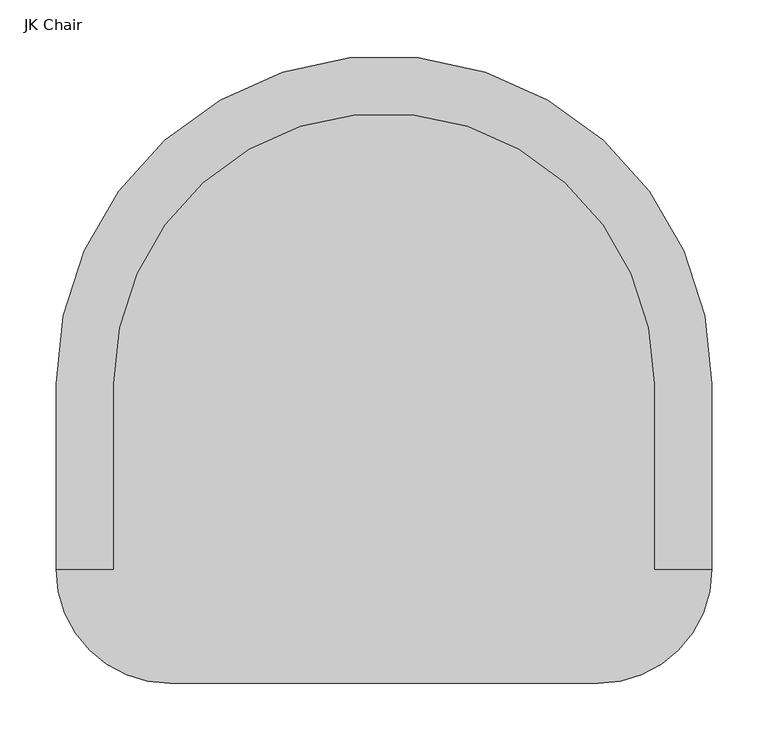
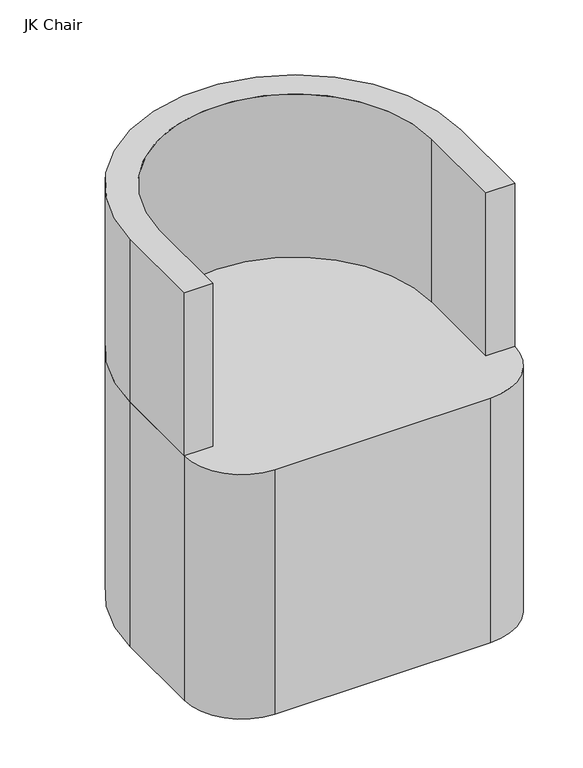
"""IFC4 building model written with IfcOpenShell, lengths in millimetres: furniture geometry, JK Chair : Recpt Chair."""

from ifc_helpers import new_model, si_unit, point, frame, frame_2d, origin, origin_with_axes, place, context, project, spatial, polyline, circle_curve, trimmed, segment, composite_curve, outline, extrude, source, transform, mapped, element, save


def jk_chair_91173c26(model_context):
    return source(origin(), model_context, "Body", "SweptSolid", [
        extrude(outline(composite_curve([segment(polyline([(-303.2426335, -131.5544704), (-354.0426335, -131.5544704), (-354.0426335, 33.5455296)]), True, "CONTINUOUS"), segment(trimmed(circle_curve(frame_2d((-61.9426335, 33.5455296)), 292.1), [point((-354.0426335, 33.5455296))], [point((230.1573665, 33.5455296))], False, "CARTESIAN"), True, "CONTINUOUS"), segment(polyline([(230.1573665, 33.5455296), (230.1573665, -131.5544704), (179.3573665, -131.5544704), (179.3573665, 33.5455296)]), True, "CONTINUOUS"), segment(trimmed(circle_curve(frame_2d((-61.9426335, 33.5455296)), 241.3), [point((179.3573665, 33.5455296))], [point((-303.2426335, 33.5455296))], True, "CARTESIAN"), True, "CONTINUOUS"), segment(polyline([(-303.2426335, 33.5455296), (-303.2426335, -131.5544704)]), True, "CONTINUOUS")], self_intersect=False)), frame((0.0, 0.0, 457.2), z_axis=(0.0, 0.0, 1.0), x_axis=(1.0, 0.0, 0.0)), (0.0, 0.0, 1.0), 304.8),
        extrude(outline(composite_curve([segment(trimmed(circle_curve(frame_2d((-61.9426335, 33.5455296)), 292.1), [point((-354.0426335, 33.5455296))], [point((230.1573665, 33.5455296))], False, "CARTESIAN"), True, "CONTINUOUS"), segment(polyline([(230.1573665, 33.5455296), (230.1573665, -131.5544704)]), True, "CONTINUOUS"), segment(trimmed(circle_curve(frame_2d((128.5573665, -131.5544704)), 101.6), [point((230.1573665, -131.5544704))], [point((128.5573665, -233.1544704))], False, "CARTESIAN"), True, "CONTINUOUS"), segment(polyline([(128.5573665, -233.1544704), (-252.4426335, -233.1544704)]), True, "CONTINUOUS"), segment(trimmed(circle_curve(frame_2d((-252.4426335, -131.5544704)), 101.6), [point((-252.4426335, -233.1544704))], [point((-354.0426335, -131.5544704))], False, "CARTESIAN"), True, "CONTINUOUS"), segment(polyline([(-354.0426335, -131.5544704), (-354.0426335, 33.5455296)]), True, "CONTINUOUS")], self_intersect=False)), origin_with_axes(), (0.0, 0.0, 1.0), 457.2),
    ])


if __name__ == "__main__":
    model = new_model("IFC4")
    model_context = context("Model", 3, world=origin())
    ifc_project = project(units=[si_unit("LENGTHUNIT", "METRE", prefix="MILLI")], contexts=[model_context])
    site = spatial("IfcSite", under=ifc_project)
    building = spatial("IfcBuilding", under=site)
    placement = place(None, origin())
    jk_chair_shape = jk_chair_91173c26(model_context)
    element("IfcFurniture", 1, ObjectType="JK Chair : Recpt Chair", at=placement, inside=building, context=model_context, shape_type="MappedRepresentation", body=[
        mapped(jk_chair_shape, transform((0.0, 0.0, 0.0), x_axis=(1.0, 0.0, 0.0), y_axis=(0.0, 1.0, 0.0), z_axis=(0.0, 0.0, 1.0))),
    ])
    save(model, "model.ifc")

# Revit data of these elements
# Type "JK Chair : Recpt Chair"
#   Width = 1' - 11"
#   Seat Height = 1' - 6"
#   Depth = 1' - 9"
#   Corner Radius = 0' - 4"
#   Back Height = 2' - 6"
#   Status [instance default] = none
#   Default Elevation = 0
